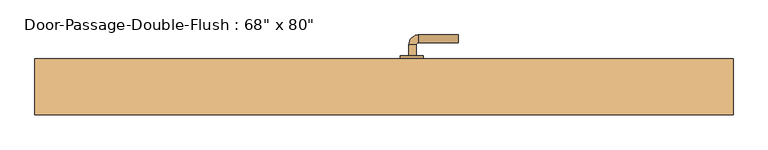
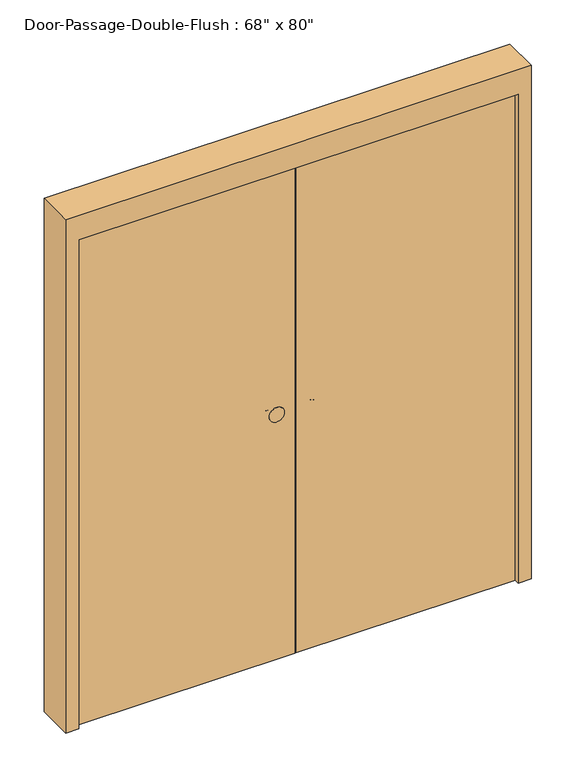
"""IFC4 building model written with IfcOpenShell, lengths in millimetres: door geometry."""

from ifc_helpers import new_model, si_unit, point, frame, frame_2d, origin, origin_with_axes, place, context, project, spatial, polyline, circle_curve, ellipse_curve, trimmed, segment, composite_curve, outline, extrude, faceted_brep, source, transform, mapped, element, save
from ifc_brep_helpers import plane_surface, cylinder_surface, revolved_surface, advanced_brep


def door_efda3cbc(model_context):
    return source(origin(), model_context, "Body", "SolidModel", [
        advanced_brep(
        [(-65.009375, 155.5125, 1016.0), (-85.009375, 155.5125, 1016.0), (-65.009375, 125.5125, 1016.0), (-85.009375, 125.5125, 1016.0), (-90.009375, 120.5125, 1016.0), (-90.009375, 100.5125, 1016.0), (-195.009375, 100.5125, 1016.0), (-195.009375, 120.5125, 1016.0)],
        [
            (0, 1, circle_curve(frame((-75.009375, 155.5125, 1016.0), z_axis=(0.0, 1.0, 0.0), x_axis=(-1.0, 0.0, 0.0)), 10.0)),
            (1, 0, circle_curve(frame((-75.009375, 155.5125, 1016.0), z_axis=(0.0, 1.0, 0.0), x_axis=(-1.0, 0.0, 0.0)), 10.0)),
            (0, 2),
            (2, 3, circle_curve(frame((-75.009375, 125.5125, 1016.0), z_axis=(0.0, 1.0, 0.0), x_axis=(-1.0, 0.0, 0.0)), 10.0)),
            (3, 1),
            (3, 2, circle_curve(frame((-75.009375, 125.5125, 1016.0), z_axis=(0.0, 1.0, 0.0), x_axis=(-1.0, 0.0, 0.0)), 10.0)),
            (4, 3, circle_curve(frame((-90.009375, 125.5125, 1016.0), z_axis=(0.0, 0.0, 1.0), x_axis=(1.0, 0.0, 0.0)), 5.0)),
            (2, 5, circle_curve(frame((-90.009375, 125.5125, 1016.0), z_axis=(0.0, 0.0, -1.0), x_axis=(1.0, 0.0, 0.0)), 25.0)),
            (5, 4, circle_curve(frame((-90.009375, 110.5125, 1016.0), z_axis=(1.0, 0.0, 0.0), x_axis=(0.0, 1.0, 0.0)), 10.0)),
            (4, 5, circle_curve(frame((-90.009375, 110.5125, 1016.0), z_axis=(1.0, 0.0, 0.0), x_axis=(0.0, 1.0, 0.0)), 10.0)),
            (6, 7, circle_curve(frame((-195.009375, 110.5125, 1016.0), z_axis=(-1.0, 0.0, 0.0), x_axis=(0.0, 1.0, 0.0)), 10.0)),
            (7, 6, circle_curve(frame((-195.009375, 110.5125, 1016.0), z_axis=(-1.0, 0.0, 0.0), x_axis=(0.0, 1.0, 0.0)), 10.0)),
            (5, 6),
            (7, 4),
        ],
        [
            plane_surface(frame((-75.009375, 155.5125, 1016.0), z_axis=(0.0, 1.0, 0.0), x_axis=(0.0, 0.0, 1.0))),
            cylinder_surface(frame((-75.009375, 155.5125, 1016.0), z_axis=(0.0, 1.0, 0.0), x_axis=(-1.0, 0.0, 0.0)), 10.0),
            revolved_surface(trimmed(ellipse_curve(frame((-75.009375, 125.5125, 1016.0), z_axis=(0.0, 1.0, 0.0), x_axis=(-1.0, 0.0, 0.0)), 10.0, 10.0), [point((-65.009375, 125.5125, 1016.0))], [point((-85.009375, 125.5125, 1016.0))], True, "CARTESIAN"), (-90.009375, 125.5125, 1016.0), (0.0, 0.0, -1.0)),
            revolved_surface(trimmed(ellipse_curve(frame((-75.009375, 125.5125, 1016.0), z_axis=(0.0, 1.0, 0.0), x_axis=(-1.0, 0.0, 0.0)), 10.0, 10.0), [point((-85.009375, 125.5125, 1016.0))], [point((-65.009375, 125.5125, 1016.0))], True, "CARTESIAN"), (-90.009375, 125.5125, 1016.0), (0.0, 0.0, -1.0)),
            plane_surface(frame((-195.009375, 110.5125, 1016.0), z_axis=(-1.0, 0.0, 0.0), x_axis=(0.0, 0.0, 1.0))),
            cylinder_surface(frame((-90.009375, 110.5125, 1016.0), z_axis=(1.0, 0.0, 0.0), x_axis=(0.0, 1.0, 0.0)), 10.0),
        ],
        [
            (0, [[1, 2]]),
            (1, [[-1, 3, 4, 5]]),
            (1, [[-2, -5, 6, -3]]),
            (2, [[7, -4, 8, 9]]),
            (3, [[-8, -6, -7, 10]]),
            (4, [[11, 12]]),
            (5, [[-9, 13, -12, 14]]),
            (5, [[-10, -14, -11, -13]]),
        ],
    ),
        extrude(outline(composite_curve([segment(trimmed(circle_curve(frame_2d((1016.0, -72.509375)), 30.0), [point((1016.0, -42.509375))], [point((1016.0, -102.509375))], False, "CARTESIAN"), True, "CONTINUOUS"), segment(trimmed(circle_curve(frame_2d((1016.0, -72.509375)), 30.0), [point((1016.0, -102.509375))], [point((1016.0, -42.509375))], False, "CARTESIAN"), True, "CONTINUOUS")], self_intersect=False)), frame((0.0, 155.5125, 0.0), z_axis=(0.0, 1.0, 0.0), x_axis=(0.0, 0.0, 1.0)), (0.0, 0.0, 1.0), 8.0),
        advanced_brep(
        [(-65.009375, 90.55, 1016.0), (-85.009375, 90.55, 1016.0), (-85.009375, 120.55, 1016.0), (-65.009375, 120.55, 1016.0), (-90.009375, 125.55, 1016.0), (-90.009375, 145.55, 1016.0), (-195.009375, 145.55, 1016.0), (-195.009375, 125.55, 1016.0)],
        [
            (0, 1, circle_curve(frame((-75.009375, 90.55, 1016.0), z_axis=(0.0, -1.0, 0.0), x_axis=(-1.0, 0.0, 0.0)), 10.0)),
            (1, 0, circle_curve(frame((-75.009375, 90.55, 1016.0), z_axis=(0.0, -1.0, 0.0), x_axis=(-1.0, 0.0, 0.0)), 10.0)),
            (1, 2),
            (2, 3, circle_curve(frame((-75.009375, 120.55, 1016.0), z_axis=(0.0, -1.0, 0.0), x_axis=(-1.0, 0.0, 0.0)), 10.0)),
            (3, 0),
            (3, 2, circle_curve(frame((-75.009375, 120.55, 1016.0), z_axis=(0.0, -1.0, 0.0), x_axis=(-1.0, 0.0, 0.0)), 10.0)),
            (4, 5, circle_curve(frame((-90.009375, 135.55, 1016.0), z_axis=(1.0, 0.0, 0.0), x_axis=(0.0, -1.0, 0.0)), 10.0)),
            (5, 3, circle_curve(frame((-90.009375, 120.55, 1016.0), z_axis=(0.0, 0.0, -1.0), x_axis=(1.0, 0.0, 0.0)), 25.0)),
            (2, 4, circle_curve(frame((-90.009375, 120.55, 1016.0), z_axis=(0.0, 0.0, 1.0), x_axis=(1.0, 0.0, 0.0)), 5.0)),
            (5, 4, circle_curve(frame((-90.009375, 135.55, 1016.0), z_axis=(1.0, 0.0, 0.0), x_axis=(0.0, -1.0, 0.0)), 10.0)),
            (6, 7, circle_curve(frame((-195.009375, 135.55, 1016.0), z_axis=(-1.0, 0.0, 0.0), x_axis=(0.0, -1.0, 0.0)), 10.0)),
            (7, 6, circle_curve(frame((-195.009375, 135.55, 1016.0), z_axis=(-1.0, 0.0, 0.0), x_axis=(0.0, -1.0, 0.0)), 10.0)),
            (4, 7),
            (6, 5),
        ],
        [
            plane_surface(frame((-75.009375, 90.55, 1016.0), z_axis=(0.0, -1.0, 0.0), x_axis=(0.0, 0.0, 1.0))),
            cylinder_surface(frame((-75.009375, 90.55, 1016.0), z_axis=(0.0, -1.0, 0.0), x_axis=(-1.0, 0.0, 0.0)), 10.0),
            revolved_surface(trimmed(ellipse_curve(frame((-75.009375, 120.55, 1016.0), z_axis=(0.0, 1.0, 0.0), x_axis=(-1.0, 0.0, 0.0)), 10.0, 10.0), [point((-65.009375, 120.55, 1016.0))], [point((-85.009375, 120.55, 1016.0))], True, "CARTESIAN"), (-90.009375, 120.55, 1016.0), (0.0, 0.0, -1.0)),
            revolved_surface(trimmed(ellipse_curve(frame((-75.009375, 120.55, 1016.0), z_axis=(0.0, 1.0, 0.0), x_axis=(-1.0, 0.0, 0.0)), 10.0, 10.0), [point((-85.009375, 120.55, 1016.0))], [point((-65.009375, 120.55, 1016.0))], True, "CARTESIAN"), (-90.009375, 120.55, 1016.0), (0.0, 0.0, -1.0)),
            plane_surface(frame((-195.009375, 135.55, 1016.0), z_axis=(-1.0, 0.0, 0.0), x_axis=(0.0, 0.0, 1.0))),
            cylinder_surface(frame((-90.009375, 135.55, 1016.0), z_axis=(1.0, 0.0, 0.0), x_axis=(0.0, -1.0, 0.0)), 10.0),
        ],
        [
            (0, [[1, 2]]),
            (1, [[3, 4, 5, -2]]),
            (1, [[-5, 6, -3, -1]]),
            (2, [[7, 8, -4, 9]]),
            (3, [[10, -9, -6, -8]]),
            (4, [[11, 12]]),
            (5, [[13, -11, 14, -7]]),
            (5, [[-14, -12, -13, -10]]),
        ],
    ),
        extrude(outline(composite_curve([segment(trimmed(circle_curve(frame_2d((1016.0, -72.509375)), 30.0), [point((1016.0, -42.509375))], [point((1016.0, -102.509375))], False, "CARTESIAN"), True, "CONTINUOUS"), segment(trimmed(circle_curve(frame_2d((1016.0, -72.509375)), 30.0), [point((1016.0, -102.509375))], [point((1016.0, -42.509375))], False, "CARTESIAN"), True, "CONTINUOUS")], self_intersect=False)), frame((0.0, 82.55, 0.0), z_axis=(0.0, 1.0, 0.0), x_axis=(0.0, 0.0, 1.0)), (0.0, 0.0, 1.0), 8.0),
        advanced_brep(
        [(65.009375, 155.5125, 1016.0), (85.009375, 155.5125, 1016.0), (85.009375, 125.5125, 1016.0), (65.009375, 125.5125, 1016.0), (90.009375, 120.5125, 1016.0), (90.009375, 100.5125, 1016.0), (195.009375, 100.5125, 1016.0), (195.009375, 120.5125, 1016.0)],
        [
            (0, 1, circle_curve(frame((75.009375, 155.5125, 1016.0), z_axis=(0.0, 1.0, 0.0), x_axis=(1.0, 0.0, 0.0)), 10.0)),
            (1, 0, circle_curve(frame((75.009375, 155.5125, 1016.0), z_axis=(0.0, 1.0, 0.0), x_axis=(1.0, 0.0, 0.0)), 10.0)),
            (1, 2),
            (2, 3, circle_curve(frame((75.009375, 125.5125, 1016.0), z_axis=(0.0, 1.0, 0.0), x_axis=(1.0, 0.0, 0.0)), 10.0)),
            (3, 0),
            (3, 2, circle_curve(frame((75.009375, 125.5125, 1016.0), z_axis=(0.0, 1.0, 0.0), x_axis=(1.0, 0.0, 0.0)), 10.0)),
            (4, 5, circle_curve(frame((90.009375, 110.5125, 1016.0), z_axis=(-1.0, 0.0, 0.0), x_axis=(0.0, 1.0, 0.0)), 10.0)),
            (5, 3, circle_curve(frame((90.009375, 125.5125, 1016.0), z_axis=(0.0, 0.0, -1.0), x_axis=(-1.0, 0.0, 0.0)), 25.0)),
            (2, 4, circle_curve(frame((90.009375, 125.5125, 1016.0), z_axis=(0.0, 0.0, 1.0), x_axis=(-1.0, 0.0, 0.0)), 5.0)),
            (5, 4, circle_curve(frame((90.009375, 110.5125, 1016.0), z_axis=(-1.0, 0.0, 0.0), x_axis=(0.0, 1.0, 0.0)), 10.0)),
            (6, 7, circle_curve(frame((195.009375, 110.5125, 1016.0), z_axis=(1.0, 0.0, 0.0), x_axis=(0.0, 1.0, 0.0)), 10.0)),
            (7, 6, circle_curve(frame((195.009375, 110.5125, 1016.0), z_axis=(1.0, 0.0, 0.0), x_axis=(0.0, 1.0, 0.0)), 10.0)),
            (4, 7),
            (6, 5),
        ],
        [
            plane_surface(frame((75.009375, 155.5125, 1016.0), z_axis=(0.0, 1.0, 0.0), x_axis=(0.0, 0.0, 1.0))),
            cylinder_surface(frame((75.009375, 155.5125, 1016.0), z_axis=(0.0, 1.0, 0.0), x_axis=(1.0, 0.0, 0.0)), 10.0),
            revolved_surface(trimmed(ellipse_curve(frame((75.009375, 125.5125, 1016.0), z_axis=(0.0, -1.0, 0.0), x_axis=(1.0, 0.0, 0.0)), 10.0, 10.0), [point((65.009375, 125.5125, 1016.0))], [point((85.009375, 125.5125, 1016.0))], True, "CARTESIAN"), (90.009375, 125.5125, 1016.0), (0.0, 0.0, -1.0)),
            revolved_surface(trimmed(ellipse_curve(frame((75.009375, 125.5125, 1016.0), z_axis=(0.0, -1.0, 0.0), x_axis=(1.0, 0.0, 0.0)), 10.0, 10.0), [point((85.009375, 125.5125, 1016.0))], [point((65.009375, 125.5125, 1016.0))], True, "CARTESIAN"), (90.009375, 125.5125, 1016.0), (0.0, 0.0, -1.0)),
            plane_surface(frame((195.009375, 110.5125, 1016.0), z_axis=(1.0, 0.0, 0.0), x_axis=(0.0, 0.0, 1.0))),
            cylinder_surface(frame((90.009375, 110.5125, 1016.0), z_axis=(-1.0, 0.0, 0.0), x_axis=(0.0, 1.0, 0.0)), 10.0),
        ],
        [
            (0, [[1, 2]]),
            (1, [[3, 4, 5, -2]]),
            (1, [[-5, 6, -3, -1]]),
            (2, [[7, 8, -4, 9]]),
            (3, [[10, -9, -6, -8]]),
            (4, [[11, 12]]),
            (5, [[13, -11, 14, -7]]),
            (5, [[-14, -12, -13, -10]]),
        ],
    ),
        extrude(outline(composite_curve([segment(trimmed(circle_curve(frame_2d((1016.0, 72.509375)), 30.0), [point((1016.0, 42.509375))], [point((1016.0, 102.509375))], False, "CARTESIAN"), True, "CONTINUOUS"), segment(trimmed(circle_curve(frame_2d((1016.0, 72.509375)), 30.0), [point((1016.0, 102.509375))], [point((1016.0, 42.509375))], False, "CARTESIAN"), True, "CONTINUOUS")], self_intersect=False)), frame((0.0, 155.5125, 0.0), z_axis=(0.0, 1.0, 0.0), x_axis=(0.0, 0.0, 1.0)), (0.0, 0.0, 1.0), 8.0),
        advanced_brep(
        [(65.009375, 215.9625, 1016.0), (85.009375, 215.9625, 1016.0), (65.009375, 245.9625, 1016.0), (85.009375, 245.9625, 1016.0), (90.009375, 250.9625, 1016.0), (90.009375, 270.9625, 1016.0), (195.009375, 270.9625, 1016.0), (195.009375, 250.9625, 1016.0)],
        [
            (0, 1, circle_curve(frame((75.009375, 215.9625, 1016.0), z_axis=(0.0, -1.0, 0.0), x_axis=(1.0, 0.0, 0.0)), 10.0)),
            (1, 0, circle_curve(frame((75.009375, 215.9625, 1016.0), z_axis=(0.0, -1.0, 0.0), x_axis=(1.0, 0.0, 0.0)), 10.0)),
            (0, 2),
            (2, 3, circle_curve(frame((75.009375, 245.9625, 1016.0), z_axis=(0.0, -1.0, 0.0), x_axis=(1.0, 0.0, 0.0)), 10.0)),
            (3, 1),
            (3, 2, circle_curve(frame((75.009375, 245.9625, 1016.0), z_axis=(0.0, -1.0, 0.0), x_axis=(1.0, 0.0, 0.0)), 10.0)),
            (4, 3, circle_curve(frame((90.009375, 245.9625, 1016.0), z_axis=(0.0, 0.0, 1.0), x_axis=(-1.0, 0.0, 0.0)), 5.0)),
            (2, 5, circle_curve(frame((90.009375, 245.9625, 1016.0), z_axis=(0.0, 0.0, -1.0), x_axis=(-1.0, 0.0, 0.0)), 25.0)),
            (5, 4, circle_curve(frame((90.009375, 260.9625, 1016.0), z_axis=(-1.0, 0.0, 0.0), x_axis=(0.0, -1.0, 0.0)), 10.0)),
            (4, 5, circle_curve(frame((90.009375, 260.9625, 1016.0), z_axis=(-1.0, 0.0, 0.0), x_axis=(0.0, -1.0, 0.0)), 10.0)),
            (6, 7, circle_curve(frame((195.009375, 260.9625, 1016.0), z_axis=(1.0, 0.0, 0.0), x_axis=(0.0, -1.0, 0.0)), 10.0)),
            (7, 6, circle_curve(frame((195.009375, 260.9625, 1016.0), z_axis=(1.0, 0.0, 0.0), x_axis=(0.0, -1.0, 0.0)), 10.0)),
            (5, 6),
            (7, 4),
        ],
        [
            plane_surface(frame((75.009375, 215.9625, 1016.0), z_axis=(0.0, -1.0, 0.0), x_axis=(0.0, 0.0, 1.0))),
            cylinder_surface(frame((75.009375, 215.9625, 1016.0), z_axis=(0.0, -1.0, 0.0), x_axis=(1.0, 0.0, 0.0)), 10.0),
            revolved_surface(trimmed(ellipse_curve(frame((75.009375, 245.9625, 1016.0), z_axis=(0.0, -1.0, 0.0), x_axis=(1.0, 0.0, 0.0)), 10.0, 10.0), [point((65.009375, 245.9625, 1016.0))], [point((85.009375, 245.9625, 1016.0))], True, "CARTESIAN"), (90.009375, 245.9625, 1016.0), (0.0, 0.0, -1.0)),
            revolved_surface(trimmed(ellipse_curve(frame((75.009375, 245.9625, 1016.0), z_axis=(0.0, -1.0, 0.0), x_axis=(1.0, 0.0, 0.0)), 10.0, 10.0), [point((85.009375, 245.9625, 1016.0))], [point((65.009375, 245.9625, 1016.0))], True, "CARTESIAN"), (90.009375, 245.9625, 1016.0), (0.0, 0.0, -1.0)),
            plane_surface(frame((195.009375, 260.9625, 1016.0), z_axis=(1.0, 0.0, 0.0), x_axis=(0.0, 0.0, 1.0))),
            cylinder_surface(frame((90.009375, 260.9625, 1016.0), z_axis=(-1.0, 0.0, 0.0), x_axis=(0.0, -1.0, 0.0)), 10.0),
        ],
        [
            (0, [[1, 2]]),
            (1, [[-1, 3, 4, 5]]),
            (1, [[-2, -5, 6, -3]]),
            (2, [[7, -4, 8, 9]]),
            (3, [[-8, -6, -7, 10]]),
            (4, [[11, 12]]),
            (5, [[-9, 13, -12, 14]]),
            (5, [[-10, -14, -11, -13]]),
        ],
    ),
        extrude(outline(composite_curve([segment(trimmed(circle_curve(frame_2d((1016.0, 72.509375)), 30.0), [point((1016.0, 42.509375))], [point((1016.0, 102.509375))], False, "CARTESIAN"), True, "CONTINUOUS"), segment(trimmed(circle_curve(frame_2d((1016.0, 72.509375)), 30.0), [point((1016.0, 102.509375))], [point((1016.0, 42.509375))], False, "CARTESIAN"), True, "CONTINUOUS")], self_intersect=False)), frame((0.0, 207.9625, 0.0), z_axis=(0.0, 1.0, 0.0), x_axis=(0.0, 0.0, 1.0)), (0.0, 0.0, 1.0), 8.0),
        faceted_brep([(863.6, 158.75, 0.0), (863.6, 207.9625, 0.0), (914.4, 207.9625, 0.0), (914.4, 61.9125, 0.0), (863.6, 61.9125, 0.0), (863.6, 111.125, 0.0), (847.725, 111.125, 0.0), (847.725, 158.75, 0.0), (863.6, 158.75, 2032.0), (863.6, 207.9625, 2032.0), (-863.6, 207.9625, 2032.0), (-863.6, 207.9625, 0.0), (-914.4, 207.9625, 0.0), (-914.4, 207.9625, 2133.6), (914.4, 207.9625, 2133.6), (914.4, 61.9125, 2133.6), (-914.4, 61.9125, 2133.6), (-914.4, 61.9125, 0.0), (-863.6, 61.9125, 0.0), (-863.6, 61.9125, 2032.0), (863.6, 61.9125, 2032.0), (863.6, 111.125, 2032.0), (-863.6, 111.125, 2032.0), (-863.6, 111.125, 0.0), (-847.725, 111.125, 0.0), (-847.725, 111.125, 2016.125), (847.725, 111.125, 2016.125), (847.725, 158.75, 2016.125), (-847.725, 158.75, 2016.125), (-847.725, 158.75, 0.0), (-863.6, 158.75, 0.0), (-863.6, 158.75, 2032.0)], [[[0, 1, 2, 3, 4, 5, 6, 7]], [[1, 0, 8, 9]], [[2, 1, 9, 10, 11, 12, 13, 14]], [[3, 2, 14, 15]], [[4, 3, 15, 16, 17, 18, 19, 20]], [[5, 4, 20, 21]], [[6, 5, 21, 22, 23, 24, 25, 26]], [[7, 6, 26, 27]], [[0, 7, 27, 28, 29, 30, 31, 8]], [[9, 8, 31, 10]], [[20, 19, 22, 21]], [[26, 25, 28, 27]], [[12, 11, 30, 29, 24, 23, 18, 17]], [[11, 10, 31, 30]], [[13, 12, 17, 16]], [[19, 18, 23, 22]], [[25, 24, 29, 28]], [[15, 14, 13, 16]]]),
        extrude(outline(polyline([(863.6, 82.55), (1.5875, 82.55), (1.5875, 163.5125), (863.6, 163.5125), (863.6, 82.55)])), origin_with_axes(), (0.0, 0.0, 1.0), 2032.0),
        extrude(outline(polyline([(-1.5875, 82.55), (-863.6, 82.55), (-863.6, 163.5125), (-1.5875, 163.5125), (-1.5875, 82.55)])), origin_with_axes(), (0.0, 0.0, 1.0), 2032.0),
    ])


if __name__ == "__main__":
    model = new_model("IFC4")
    model_context = context("Model", 3, world=origin())
    ifc_project = project(units=[si_unit("LENGTHUNIT", "METRE", prefix="MILLI")], contexts=[model_context])
    site = spatial("IfcSite", under=ifc_project)
    building = spatial("IfcBuilding", under=site)
    placement = place(None, origin())
    door_shape = door_efda3cbc(model_context)
    element("IfcDoor", 1, ObjectType="Door-Passage-Double-Flush : 68\" x 80\"", at=placement, inside=building, context=model_context, shape_type="MappedRepresentation", body=[
        mapped(door_shape, transform((0.0, 0.0, 0.0), x_axis=(1.0, 0.0, 0.0), y_axis=(0.0, 1.0, 0.0), z_axis=(0.0, 0.0, 1.0))),
    ])
    save(model, "model.ifc")

# Revit data of these elements
# Type "Door-Passage-Double-Flush : 68\" x 80\""
#   Type Mark = "66"
#   Assembly Code = "B2030200"
#   Analytic Construction = "Metal"
#   Thickness = 0' - 1 3/4"
#   Thermal Resistance (R) = 1.5338 (h·ft²·°F)/BTU
#   Swing Angle [instance default] = 90.00°
#   Strike Height = 3' - 4"
#   SinglePanelWidth = 2' - 10"
#   Rough Width [instance default] = 6' - 0"
#   Rough Height [instance default] = 7' - 0"
#   MFOpeningHeight [instance default] = 0' - 4"
#   MFOpeningWidth [instance default] = 0' - 4"
#   Inset Calculate [instance default] = 0' - 4"
#   Masonry Inset [instance default] = 0' - 1"
#   Height = 6' - 8"
#   Width = 5' - 8"
#   Heat Transfer Coefficient (U) = 0.6520 BTU/(h·ft²·°F)
#   Masonry Frame Depth = 0' - 5 3/4"
#   Masonry Frame [instance default] = yes
#   Function = 1
#   Dry Wall Frame [instance default] = no
#   Panel Material = Metal Door - Brindle
#   Frame Material = Metal - Painted - Grey
#   Door Handle Material = Metal - Aluminium
#   Visual Light Transmittance = 0
#   Solar Heat Gain Coefficient = 0
#   Wall Closure = (empty or 0)
# Element 1 (IfcDoor, "Door-Passage-Double-Flush : 68\" x 80\"")
#   Materials on its faces: "Metal - Aluminium", "Metal - Painted - Grey", "Metal Door - Brindle"
# Materials
#   "Metal Door - Brindle": class "Paint", colour RGB 164 133 98, transparency 0
#   "Metal - Painted - Grey": class "Paint", colour RGB 104 104 104, transparency 0
#   "Metal - Aluminium": class "Metal", colour RGB 244 244 244, transparency 0
